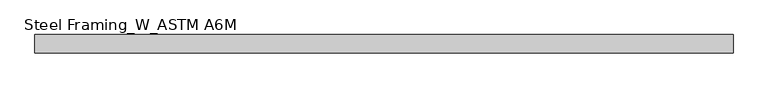
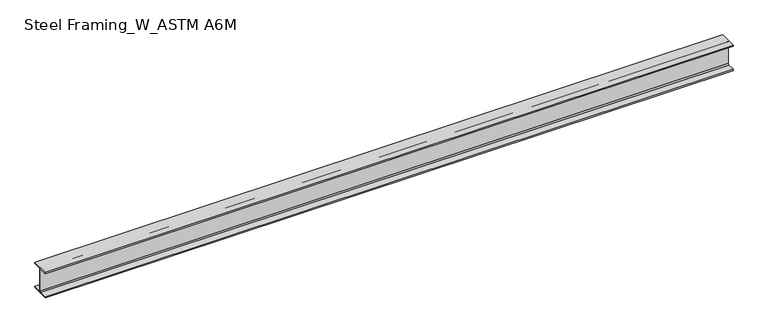
"""IFC4 building model written with IfcOpenShell, lengths in millimetres: beam geometry, Steel Framing_W_ASTM A6M : H_SB_AR_S02_W310x60_G4."""

from ifc_helpers import new_model, si_unit, point, frame, frame_2d, origin, place, context, project, spatial, polyline, circle_curve, trimmed, segment, composite_curve, outline, extrude, source, transform, mapped, element, save


def steel_framing_w_astm_a6m_83ea1368(model_context):
    return source(origin(), model_context, "Body", "SweptSolid", [
        extrude(outline(composite_curve([segment(polyline([(101.5, -137.9), (101.5, -151.0), (-101.5, -151.0), (-101.5, -137.9), (-16.545, -137.9)]), True, "CONTINUOUS"), segment(trimmed(circle_curve(frame_2d((-16.545, -125.1)), 12.8), [point((-16.545, -137.9))], [point((-3.745, -125.1))], True, "CARTESIAN"), True, "CONTINUOUS"), segment(polyline([(-3.745, -125.1), (-3.745, 125.1)]), True, "CONTINUOUS"), segment(trimmed(circle_curve(frame_2d((-16.545, 125.1)), 12.8), [point((-3.745, 125.1))], [point((-16.545, 137.9))], True, "CARTESIAN"), True, "CONTINUOUS"), segment(polyline([(-16.545, 137.9), (-101.5, 137.9), (-101.5, 151.0), (101.5, 151.0), (101.5, 137.9), (16.545, 137.9)]), True, "CONTINUOUS"), segment(trimmed(circle_curve(frame_2d((16.545, 125.1)), 12.8), [point((16.545, 137.9))], [point((3.745, 125.1))], True, "CARTESIAN"), True, "CONTINUOUS"), segment(polyline([(3.745, 125.1), (3.745, -125.1)]), True, "CONTINUOUS"), segment(trimmed(circle_curve(frame_2d((16.545, -125.1)), 12.8), [point((3.745, -125.1))], [point((16.545, -137.9))], True, "CARTESIAN"), True, "CONTINUOUS"), segment(polyline([(16.545, -137.9), (101.5, -137.9)]), True, "CONTINUOUS")], self_intersect=False)), frame((-3884.3, 0.0, 0.0), z_axis=(1.0, 0.0, 0.0), x_axis=(0.0, 1.0, 0.0)), (0.0, 0.0, 1.0), 7768.6),
    ])


if __name__ == "__main__":
    model = new_model("IFC4")
    model_context = context("Model", 3, world=origin())
    ifc_project = project(units=[si_unit("LENGTHUNIT", "METRE", prefix="MILLI")], contexts=[model_context])
    site = spatial("IfcSite", under=ifc_project)
    building = spatial("IfcBuilding", under=site)
    placement = place(None, origin())
    steel_framing_w_astm_a6m_shape = steel_framing_w_astm_a6m_83ea1368(model_context)
    element("IfcBeam", 1, ObjectType="Steel Framing_W_ASTM A6M : H_SB_AR_S02_W310x60_G4", at=placement, inside=building, context=model_context, shape_type="MappedRepresentation", body=[
        mapped(steel_framing_w_astm_a6m_shape, transform((0.0, 0.0, 0.0), x_axis=(1.0, 0.0, 0.0), y_axis=(0.0, 1.0, 0.0), z_axis=(0.0, 0.0, 1.0))),
    ])
    save(model, "model.ifc")

# Revit data of these elements
# Type "Steel Framing_W_ASTM A6M : H_SB_AR_S02_W310x60_G4"
#   Type Mark = "G4"
#   Section Name Key = "W12x40"
#   Width = 20.3 cm
#   Web Thickness = 0.749 cm
#   Web Fillet = 1.28 cm
#   Warping Constant = 387000.0 cm⁶
#   Torsional Moment of Inertia = 37.70 cm⁴
#   Section Area = 75.5 cm²
#   Plastic Modulus weak axis = 275.0 cm³
#   Plastic Modulus strong axis = 934.0 cm³
#   Perimeter = 1.38 m²/m
#   Nominal Weight = 60.00 kgf/m
#   Moment of Inertia weak axis = 1840.00 cm⁴
#   Moment of Inertia strong axis = 12800.00 cm⁴
#   Height = 30.2 cm
#   Flange Thickness = 1.31 cm
#   Elastic Modulus weak axis = 180.0 cm³
#   Elastic Modulus strong axis = 844.0 cm³
#   Centroid Vertical = 15.1 cm
#   Centroid Horizontal = 10.15 cm
#   Length [instance default] = 1500 mm
#   Structural Material [instance default] = Steel, 45-345
#   Bolt Spacing = 0
#   Assembly Code = ""
# Element 1 (IfcBeam, "Steel Framing_W_ASTM A6M : H_SB_AR_S02_W310x60_G4")
#   Materials on its faces: "Steel, 45-345"
# Materials
#   "Steel, 45-345": class "Metal", colour RGB 189 187 185, transparency 0, Description = "Steel 345 MPa", Cost = 0
